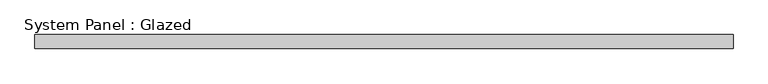
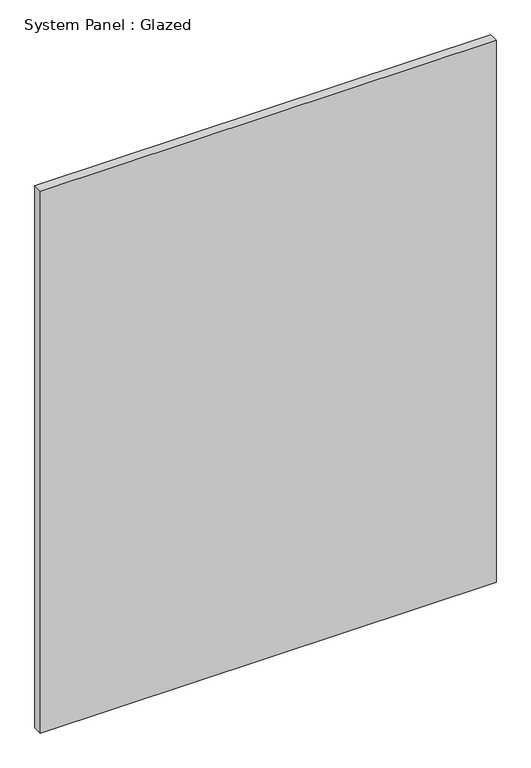
"""IFC4 building model written with IfcOpenShell, lengths in millimetres: plate geometry, System Panel : Glazed."""

import ifcopenshell
import ifcopenshell.guid

model = None  # the IFC model being written
_history = None  # IfcOwnerHistory: only IFC2X3 demands one
_inside = {}  # id of a spatial element -> (the spatial element, [elements in it])
_under = {}  # id of a project, library or spatial element -> (it, [spatial elements below it])
_declared = {}  # id of a project -> (the project, [libraries it declares])
_typed = {}  # id of a type object -> (the type object, [elements of that type])
_made_of = {}  # id of a material, layer set ... -> (it, [elements and type objects made of it])


def new_model(schema):
    """Start an empty IFC model of exactly this schema.

    Asked for "IFC4X3", IfcOpenShell would pick the latest addendum, in which some entities
    have other attributes; the version numbers below select the first issue.
    IFC2X3 requires an IfcOwnerHistory on every rooted entity: one is made here for all.
    """
    global model, _history
    if schema == "IFC4X3":
        model = ifcopenshell.file(schema_version=(4, 3, 0, 0))
    else:
        model = ifcopenshell.file(schema=schema)
    _inside.clear()
    _under.clear()
    _declared.clear()
    _typed.clear()
    _made_of.clear()
    _history = None
    if model.schema == "IFC2X3":
        org = make("IfcOrganization", Name="unknown")
        user = make(
            "IfcPersonAndOrganization",
            ThePerson=make("IfcPerson", FamilyName="unknown"),
            TheOrganization=org,
        )
        app = make(
            "IfcApplication",
            ApplicationDeveloper=org,
            Version="unknown",
            ApplicationFullName="unknown",
            ApplicationIdentifier="unknown",
        )
        _history = make(
            "IfcOwnerHistory",
            OwningUser=user,
            OwningApplication=app,
            ChangeAction="ADDED",
            CreationDate=0,
        )
    return model


def make(cls, **values):
    """One entity of the class cls with the attributes given. An attribute that is None is left unset."""
    return model.create_entity(
        cls, **{name: value for name, value in values.items() if value is not None}
    )


def rooted(cls, **values):
    """An entity with a GlobalId (a new one), such as an element, a storey or a relation."""
    return make(cls, GlobalId=ifcopenshell.guid.new(), OwnerHistory=_history, **values)


def si_unit(unit_type, name, prefix=None):
    """IfcSIUnit, for example si_unit("LENGTHUNIT", "METRE", prefix="MILLI")."""
    return make("IfcSIUnit", UnitType=unit_type, Prefix=prefix, Name=name)


def assignment(units):
    """IfcUnitAssignment: the units of a project."""
    return None if units is None else make("IfcUnitAssignment", Units=units)


def point(xyz):
    """IfcCartesianPoint."""
    return None if xyz is None else make("IfcCartesianPoint", Coordinates=xyz)


def direction(xyz):
    """IfcDirection."""
    return None if xyz is None else make("IfcDirection", DirectionRatios=xyz)


def frame(location, z_axis=None, x_axis=None):
    """IfcAxis2Placement3D, a coordinate frame: its origin and axes. An axis left out is left unset."""
    return make(
        "IfcAxis2Placement3D",
        Location=point(location),
        Axis=direction(z_axis),
        RefDirection=direction(x_axis),
    )


def origin():
    """The frame at (0, 0, 0) with its axes left unset."""
    return frame((0.0, 0.0, 0.0))


def origin_with_axes():
    """The frame at (0, 0, 0) with the z axis (0, 0, 1) and the x axis (1, 0, 0) written out."""
    return frame((0.0, 0.0, 0.0), z_axis=(0.0, 0.0, 1.0), x_axis=(1.0, 0.0, 0.0))


def place(relative_to, where):
    """IfcLocalPlacement: puts the frame where relative to a parent placement (None: the world)."""
    return make(
        "IfcLocalPlacement", PlacementRelTo=relative_to, RelativePlacement=where
    )


def context(
    kind, dimensions, precision=None, world=None, true_north=None, identifier=None
):
    """IfcGeometricRepresentationContext, for example the 3D "Model" context."""
    return make(
        "IfcGeometricRepresentationContext",
        ContextIdentifier=identifier,
        ContextType=kind,
        CoordinateSpaceDimension=dimensions,
        Precision=precision,
        WorldCoordinateSystem=world,
        TrueNorth=true_north,
    )


def project(units=None, contexts=None):
    """IfcProject with its units and contexts."""
    return rooted(
        "IfcProject",
        Name="project",
        RepresentationContexts=contexts,
        UnitsInContext=assignment(units),
    )


def spatial(cls, under=None, at=None, **own):
    """A site, building, storey or space (cls), placed at a placement, below another one or the project."""
    s = rooted(cls, ObjectPlacement=at, **own)
    if under is not None:
        _under.setdefault(under.id(), (under, []))[1].append(s)
    return s


def polyline(points):
    """IfcPolyline through the points."""
    return make("IfcPolyline", Points=[point(p) for p in points])


def outline(outer, holes=None, kind="AREA"):
    """IfcArbitraryClosedProfileDef: a profile drawn as a closed curve; with holes, ...WithVoids."""
    if holes is None:
        return make("IfcArbitraryClosedProfileDef", ProfileType=kind, OuterCurve=outer)
    return make(
        "IfcArbitraryProfileDefWithVoids",
        ProfileType=kind,
        OuterCurve=outer,
        InnerCurves=holes,
    )


def extrude(swept, where, along, depth):
    """IfcExtrudedAreaSolid: the profile swept, set in the frame where, extruded along a direction by depth."""
    return make(
        "IfcExtrudedAreaSolid",
        SweptArea=swept,
        Position=where,
        ExtrudedDirection=direction(along),
        Depth=depth,
    )


def shape(context_of_items, identifier, shape_type, items):
    """IfcShapeRepresentation: the items that make up one representation, for example the "Body"."""
    return make(
        "IfcShapeRepresentation",
        ContextOfItems=context_of_items,
        RepresentationIdentifier=identifier,
        RepresentationType=shape_type,
        Items=items,
    )


def source(mapping_origin, context_of_items, identifier, shape_type, items):
    """IfcRepresentationMap: a shape defined once, which mapped items show again and again."""
    return make(
        "IfcRepresentationMap",
        MappingOrigin=mapping_origin,
        MappedRepresentation=shape(context_of_items, identifier, shape_type, items),
    )


def transform(
    local_origin,
    x_axis=None,
    y_axis=None,
    z_axis=None,
    scale=None,
    scale2=None,
    scale3=None,
    uniform=True,
):
    """IfcCartesianTransformationOperator3D, or its non-uniform kind. x_axis, y_axis, z_axis: its Axis1, 2, 3."""
    if uniform:
        return make(
            "IfcCartesianTransformationOperator3D",
            Axis1=direction(x_axis),
            Axis2=direction(y_axis),
            LocalOrigin=point(local_origin),
            Scale=scale,
            Axis3=direction(z_axis),
        )
    return make(
        "IfcCartesianTransformationOperator3DnonUniform",
        Axis1=direction(x_axis),
        Axis2=direction(y_axis),
        LocalOrigin=point(local_origin),
        Scale=scale,
        Axis3=direction(z_axis),
        Scale2=scale2,
        Scale3=scale3,
    )


def mapped(mapping_source, mapping_target):
    """IfcMappedItem: shows the shape of a source again, moved by a transform."""
    return make(
        "IfcMappedItem", MappingSource=mapping_source, MappingTarget=mapping_target
    )


def made_of(thing, what):
    """Note that an element or type object is made of a material, layer set ...; save() writes the relation."""
    if what is not None:
        _made_of.setdefault(what.id(), (what, []))[1].append(thing)
    return thing


def element(
    cls,
    number,
    at=None,
    inside=None,
    cuts=None,
    type_object=None,
    material=None,
    context=None,
    identifier="Body",
    shape_type=None,
    held_by="IfcProductDefinitionShape",
    body=None,
    shapes=None,
    **own,
):
    """One element of the class cls, such as IfcWall. Its Tag is "e" and its number.

    at: its placement. inside: the storey or other place that contains it. cuts: it is an
    opening in that element (IfcRelVoidsElement). A single representation is given by context,
    identifier, shape_type and body (its items); several are given by shapes. held_by: the class
    of the entity that holds the representations. save() writes the other relations.
    """
    e = rooted(cls, Tag="e%d" % number, ObjectPlacement=at, **own)
    if body is not None:
        shapes = [shape(context, identifier, shape_type, body)]
    if shapes is not None:
        e.Representation = make(held_by, Representations=shapes)
    if inside is not None:
        _inside.setdefault(inside.id(), (inside, []))[1].append(e)
    if cuts is not None:
        rooted(
            "IfcRelVoidsElement", RelatingBuildingElement=cuts, RelatedOpeningElement=e
        )
    if type_object is not None:
        _typed.setdefault(type_object.id(), (type_object, []))[1].append(e)
    return made_of(e, material)


def aggregate(whole, parts):
    """IfcRelAggregates: a whole, such as a stair, and the parts it consists of."""
    return rooted("IfcRelAggregates", RelatingObject=whole, RelatedObjects=parts)


def save(model, path):
    """Write the relations noted so far, then the file.

    IfcRelAggregates (storeys below a building ...), IfcRelContainedInSpatialStructure (elements
    in a storey), IfcRelDefinesByType, IfcRelAssociatesMaterial and IfcRelDeclares: one each for
    every whole, place, type object, material and project.
    """
    for whole, parts in _under.values():
        aggregate(whole, parts)
    for where, things in _inside.values():
        rooted(
            "IfcRelContainedInSpatialStructure",
            RelatedElements=things,
            RelatingStructure=where,
        )
    for kind, things in _typed.values():
        rooted("IfcRelDefinesByType", RelatedObjects=things, RelatingType=kind)
    for what, things in _made_of.values():
        rooted("IfcRelAssociatesMaterial", RelatedObjects=things, RelatingMaterial=what)
    for by, libraries in _declared.values():
        rooted("IfcRelDeclares", RelatingContext=by, RelatedDefinitions=libraries)
    model.write(path)


def system_panel_glazed_d4804bae(model_context):
    return source(origin(), model_context, "Body", "SweptSolid", [
        extrude(outline(polyline([(620.5541356, 24.5), (-620.5541356, 24.5), (-620.5541356, 49.5), (620.5541356, 49.5), (620.5541356, 24.5)])), origin_with_axes(), (0.0, 0.0, 1.0), 1560.0991456),
    ])


if __name__ == "__main__":
    model = new_model("IFC4")
    model_context = context("Model", 3, world=origin())
    ifc_project = project(units=[si_unit("LENGTHUNIT", "METRE", prefix="MILLI")], contexts=[model_context])
    site = spatial("IfcSite", under=ifc_project)
    building = spatial("IfcBuilding", under=site)
    placement = place(None, origin())
    system_panel_glazed_shape = system_panel_glazed_d4804bae(model_context)
    element("IfcPlate", 1, ObjectType="System Panel : Glazed", at=placement, inside=building, context=model_context, shape_type="MappedRepresentation", body=[
        mapped(system_panel_glazed_shape, transform((0.0, 0.0, 0.0), x_axis=(1.0, 0.0, 0.0), y_axis=(0.0, 1.0, 0.0), z_axis=(0.0, 0.0, 1.0))),
    ])
    save(model, "model.ifc")

# Revit data of these elements
# Type "System Panel : Glazed"
#   Construction Type Id = "GSP4R"
#   Analytic Construction = "1/8 in Pilkington single glazing"
#   Visual Light Transmittance = 0.9
#   Solar Heat Gain Coefficient = 0.86
#   Heat Transfer Coefficient (U) = 6.7069 W/(m²·K)
#   Define Thermal Properties by = 1
# Element 1 (IfcPlate, "System Panel : Glazed")
#   Materials on its faces: "Glass"
# Materials
#   "Glass": class "Glass", colour RGB 0 128 192, transparency 0.9, Description = "Soda Lime Glass", Cost = 0
